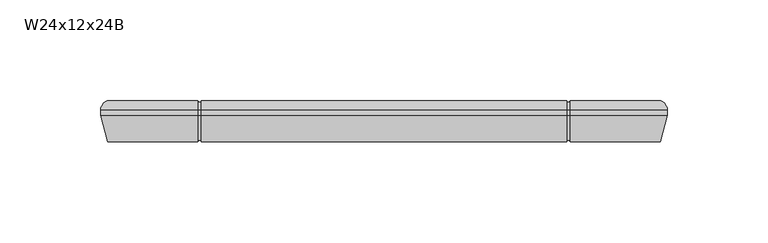
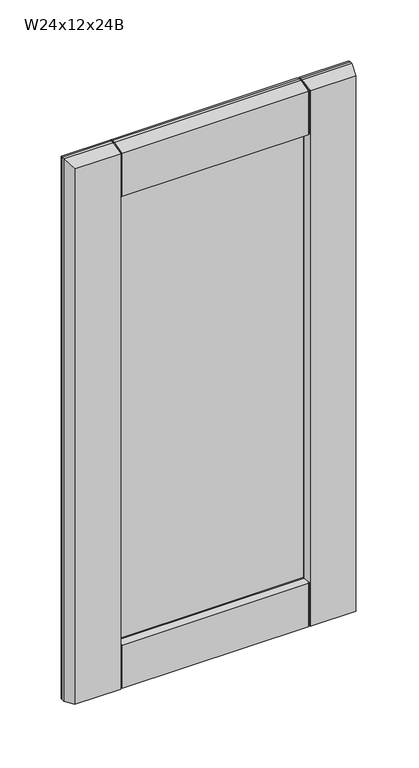
"""IFC4 building model written with IfcOpenShell, lengths in millimetres: furniture geometry, Cabinet-Wall-Merillat-Double_Door-Marlin : W24x12x24B."""

from ifc_helpers import new_model, si_unit, frame, origin, place, context, project, spatial, polyline, circle_curve, ellipse_curve, outline, extrude, source, transform, mapped, element, save
from ifc_brep_helpers import plane_surface, cylinder_surface, advanced_brep


def w24x12x24b_108fa4a6(model_context):
    return source(origin(), model_context, "Body", "SolidModel", [
        advanced_brep(
        [(541.0528392, 382.5621, 2108.2), (541.0528392, 382.5621, 1549.4), (537.9563467, 387.0325, 1552.4964925), (537.9563467, 387.0325, 2105.1035075), (541.0528392, 379.7935, 2108.2), (541.0528392, 379.7935, 1549.4), (537.5476392, 366.7125, 2104.6948), (537.5476392, 366.7125, 1552.9052), (492.8516765, 366.7125, 2059.9988372), (492.4815448, 367.50625, 2059.6287055), (490.4003857, 371.96931, 2057.5475465), (490.4003857, 371.96931, 1600.0524535), (492.4815448, 367.50625, 1597.9712945), (492.8516765, 366.7125, 1597.6011628), (491.8001552, 374.2094093, 2058.947316), (491.8001552, 374.2094093, 1598.652684), (506.1278392, 374.4595, 2073.275), (506.1278392, 374.4595, 1584.325), (506.1278392, 379.2855, 2073.275), (506.1278392, 379.2855, 1584.325), (491.8001552, 379.5355907, 2058.947316), (491.8001552, 379.5355907, 1598.652684), (490.4003857, 381.77569, 2057.5475465), (490.4003857, 381.77569, 1600.0524535), (492.4815448, 386.23875, 2059.6287055), (492.848809, 387.0263508, 2059.9959698), (492.8516765, 387.0325, 1597.6011628), (492.4815448, 386.23875, 1597.9712945), (263.1618317, 387.0325, 1552.4964925), (308.2295579, 387.0325, 1552.4964925), (308.2295579, 382.5621, 1549.4), (260.0653392, 382.5621, 1549.4), (492.848809, 382.5621, 1549.4), (492.848809, 387.0325, 1552.4964925), (491.261309, 382.5621, 1549.4), (309.8170579, 382.5621, 1549.4), (309.8170579, 387.0325, 1552.4964925), (491.261309, 387.0325, 1552.4964925), (308.2295579, 379.7935, 1549.4), (260.0653392, 379.7935, 1549.4), (492.848809, 379.7935, 1549.4), (491.261309, 379.7935, 1549.4), (309.8170579, 379.7935, 1549.4), (308.2295579, 366.7125, 1552.9052), (263.5705392, 366.7125, 1552.9052), (491.261309, 366.7125, 1552.9052), (309.8170579, 366.7125, 1552.9052), (492.848809, 366.7125, 1552.9052), (310.7177927, 371.96931, 1600.0524535), (308.6366337, 367.50625, 1597.9712945), (309.8170579, 367.50625, 1597.9712945), (309.8170579, 366.7125, 1597.6011628), (491.261309, 366.7125, 1597.6011628), (491.261309, 367.50625, 1597.9712945), (309.3180233, 374.2094093, 1598.652684), (294.9903392, 374.4595, 1584.325), (294.9903392, 379.2855, 1584.325), (309.3180233, 379.5355907, 1598.652684), (310.7177927, 381.77569, 1600.0524535), (491.261309, 386.23875, 1597.9712945), (491.261309, 387.0325, 1597.6011628), (309.8170579, 387.0325, 1597.6011628), (309.8170579, 386.23875, 1597.9712945), (308.6366337, 386.23875, 1597.9712945), (260.0653392, 382.5621, 2108.2), (263.1618317, 387.0325, 2105.1035075), (260.0653392, 379.7935, 2108.2), (263.5705392, 366.7125, 2104.6948), (308.266502, 366.7125, 1597.6011628), (310.7177927, 371.96931, 2057.5475465), (308.6366337, 367.50625, 2059.6287055), (308.266502, 366.7125, 2059.9988372), (309.3180233, 374.2094093, 2058.947316), (294.9903392, 374.4595, 2073.275), (294.9903392, 379.2855, 2073.275), (309.3180233, 379.5355907, 2058.947316), (310.7177927, 381.77569, 2057.5475465), (308.266502, 387.0325, 1597.6011628), (308.266502, 387.0325, 2059.9988372), (308.6366337, 386.23875, 2059.6287055), (492.848809, 387.0325, 2105.1035075), (492.848809, 382.5621, 2108.2), (308.2295579, 382.5621, 2108.2), (308.2295579, 387.0325, 2105.1035075), (309.8170579, 382.5621, 2108.2), (491.261309, 382.5621, 2108.2), (491.261309, 387.0325, 2105.1035075), (309.8170579, 387.0325, 2105.1035075), (492.848809, 379.7935, 2108.2), (308.2295579, 379.7935, 2108.2), (309.8170579, 379.7935, 2108.2), (491.261309, 379.7935, 2108.2), (492.848809, 366.7125, 2104.6948), (308.2295579, 366.7125, 2104.6948), (309.8170579, 366.7125, 2104.6948), (491.261309, 366.7125, 2104.6948), (309.8170579, 366.7125, 2059.9988372), (491.261309, 366.7125, 2059.9988372), (491.261309, 367.50625, 2059.6287055), (309.8170579, 367.50625, 2059.6287055), (309.8170579, 386.23875, 2059.6287055), (309.8170579, 387.0325, 2059.9988372), (491.261309, 387.0325, 2059.9988372), (491.261309, 386.23875, 2059.6287055), (309.8170579, 386.23875, 2104.9526052), (309.8170579, 382.5621, 2107.40625), (309.8170579, 379.8980037, 2107.40625), (309.8170579, 367.50625, 2104.0857412), (308.2295579, 367.50625, 2059.6287055), (308.2295579, 367.50625, 2104.0857412), (308.2295579, 379.8980037, 2107.40625), (308.2295579, 382.5621, 2107.40625), (308.2295579, 386.23875, 2104.9526052), (308.2295579, 386.23875, 2059.6287055), (492.848809, 386.23875, 2059.6287055), (492.848809, 386.23875, 2104.9526052), (492.848809, 382.5621, 2107.40625), (492.848809, 379.8980037, 2107.40625), (492.848809, 367.50625, 2104.0857412), (492.848809, 367.50625, 2059.6287055), (491.261309, 367.50625, 2104.0857412), (491.261309, 379.8980037, 2107.40625), (491.261309, 382.5621, 2107.40625), (491.261309, 386.23875, 2104.9526052), (492.848809, 367.50625, 1597.9712945), (492.848809, 367.50625, 1553.5142588), (492.848809, 379.8980037, 1550.19375), (492.848809, 382.5621, 1550.19375), (492.848809, 386.23875, 1552.6473948), (492.848809, 386.23875, 1597.9712945), (491.261309, 386.23875, 1552.6473948), (491.261309, 382.5621, 1550.19375), (491.261309, 379.8980037, 1550.19375), (491.261309, 367.50625, 1553.5142588), (309.8170579, 367.50625, 1553.5142588), (309.8170579, 379.8980037, 1550.19375), (309.8170579, 382.5621, 1550.19375), (309.8170579, 386.23875, 1552.6473948), (308.2295579, 386.23875, 1597.9712945), (308.2295579, 386.23875, 1552.6473948), (308.2295579, 382.5621, 1550.19375), (308.2295579, 379.8980037, 1550.19375), (308.2295579, 367.50625, 1553.5142588), (308.2295579, 367.50625, 1597.9712945)],
        [
            (0, 1),
            (1, 2, ellipse_curve(frame((536.2776392, 382.5621, 1554.1752), z_axis=(0.7071067811865475, 0.0, 0.7071067811865475), x_axis=(-0.7071067811865474, 0.0, 0.7071067811865476)), 6.7531526, 4.7752)),
            (2, 3),
            (3, 0, ellipse_curve(frame((536.2776392, 382.5621, 2103.4248), z_axis=(0.7071067811865475, 0.0, -0.7071067811865475), x_axis=(0.7071067811865474, 0.0, 0.7071067811865476)), 6.7531526, 4.7752)),
            (0, 4),
            (4, 5),
            (5, 1),
            (4, 6),
            (6, 7),
            (7, 5),
            (8, 9),
            (9, 10),
            (10, 11),
            (11, 12),
            (12, 13),
            (13, 8),
            (10, 14, ellipse_curve(frame((491.8276392, 372.6348492, 2058.9748), z_axis=(0.7071067811865475, 0.0, -0.7071067811865475), x_axis=(0.7071067811865474, 0.0, 0.7071067811865476)), 2.2271035, 1.5748)),
            (14, 15),
            (15, 11, ellipse_curve(frame((491.8276392, 372.6348492, 1598.6252), z_axis=(0.7071067811865475, 0.0, 0.7071067811865475), x_axis=(-0.7071067811865474, 0.0, 0.7071067811865476)), 2.2271035, 1.5748)),
            (14, 16),
            (16, 17),
            (17, 15),
            (16, 18),
            (18, 19),
            (19, 17),
            (18, 20),
            (20, 21),
            (21, 19),
            (20, 22, ellipse_curve(frame((491.8276392, 381.1101508, 2058.9748), z_axis=(0.7071067811865475, 0.0, -0.7071067811865475), x_axis=(0.7071067811865474, 0.0, 0.7071067811865476)), 2.2271035, 1.5748)),
            (22, 23),
            (23, 21, ellipse_curve(frame((491.8276392, 381.1101508, 1598.6252), z_axis=(0.7071067811865475, 0.0, 0.7071067811865475), x_axis=(-0.7071067811865474, 0.0, 0.7071067811865476)), 2.2271035, 1.5748)),
            (22, 24),
            (24, 25),
            (25, 26),
            (26, 27),
            (27, 23),
            (28, 29),
            (29, 30, circle_curve(frame((308.2295579, 382.5621, 1554.1752), z_axis=(-1.0, 0.0, 0.0), x_axis=(0.0, -1.0, 0.0)), 4.7752)),
            (30, 31),
            (31, 28, ellipse_curve(frame((264.8405392, 382.5621, 1554.1752), z_axis=(0.7071067811865475, 0.0, -0.7071067811865475), x_axis=(0.7071067811865476, 0.0, 0.7071067811865474)), 6.7531526, 4.7752)),
            (1, 32),
            (32, 33, circle_curve(frame((492.848809, 382.5621, 1554.1752), z_axis=(1.0, 0.0, 0.0), x_axis=(0.0, -1.0, 0.0)), 4.7752)),
            (33, 2),
            (34, 35),
            (35, 36, circle_curve(frame((309.8170579, 382.5621, 1554.1752), z_axis=(1.0, 0.0, 0.0), x_axis=(0.0, -1.0, 0.0)), 4.7752)),
            (36, 37),
            (37, 34, circle_curve(frame((491.261309, 382.5621, 1554.1752), z_axis=(-1.0, 0.0, 0.0), x_axis=(0.0, -1.0, 0.0)), 4.7752)),
            (30, 38),
            (38, 39),
            (39, 31),
            (5, 40),
            (40, 32),
            (41, 42),
            (42, 35),
            (34, 41),
            (38, 43),
            (43, 44),
            (44, 39),
            (45, 46),
            (46, 42),
            (41, 45),
            (7, 47),
            (47, 40),
            (48, 49),
            (49, 50),
            (50, 51),
            (51, 52),
            (52, 53),
            (53, 12),
            (11, 48),
            (15, 54),
            (54, 48, ellipse_curve(frame((309.2905392, 372.6348492, 1598.6252), z_axis=(0.7071067811865475, 0.0, -0.7071067811865475), x_axis=(0.7071067811865476, 0.0, 0.7071067811865474)), 2.2271035, 1.5748)),
            (17, 55),
            (55, 54),
            (19, 56),
            (56, 55),
            (21, 57),
            (57, 56),
            (23, 58),
            (58, 57, ellipse_curve(frame((309.2905392, 381.1101508, 1598.6252), z_axis=(0.7071067811865475, 0.0, -0.7071067811865475), x_axis=(0.7071067811865476, 0.0, 0.7071067811865474)), 2.2271035, 1.5748)),
            (27, 59),
            (59, 60),
            (60, 61),
            (61, 62),
            (62, 63),
            (63, 58),
            (31, 64),
            (64, 65, ellipse_curve(frame((264.8405392, 382.5621, 2103.4248), z_axis=(-0.7071067811865475, 0.0, -0.7071067811865475), x_axis=(0.7071067811865474, 0.0, -0.7071067811865476)), 6.7531526, 4.7752)),
            (65, 28),
            (39, 66),
            (66, 64),
            (44, 67),
            (67, 66),
            (68, 49),
            (48, 69),
            (69, 70),
            (70, 71),
            (71, 68),
            (54, 72),
            (72, 69, ellipse_curve(frame((309.2905392, 372.6348492, 2058.9748), z_axis=(-0.7071067811865475, 0.0, -0.7071067811865475), x_axis=(0.7071067811865474, 0.0, -0.7071067811865476)), 2.2271035, 1.5748)),
            (55, 73),
            (73, 72),
            (56, 74),
            (74, 73),
            (57, 75),
            (75, 74),
            (58, 76),
            (76, 75, ellipse_curve(frame((309.2905392, 381.1101508, 2058.9748), z_axis=(-0.7071067811865475, 0.0, -0.7071067811865475), x_axis=(0.7071067811865474, 0.0, -0.7071067811865476)), 2.2271035, 1.5748)),
            (63, 77),
            (77, 78),
            (78, 79),
            (79, 76),
            (3, 80),
            (80, 81, circle_curve(frame((492.848809, 382.5621, 2103.4248), z_axis=(1.0, 0.0, 0.0), x_axis=(0.0, -1.0, 0.0)), 4.7752)),
            (81, 0),
            (64, 82),
            (82, 83, circle_curve(frame((308.2295579, 382.5621, 2103.4248), z_axis=(-1.0, 0.0, 0.0), x_axis=(0.0, -1.0, 0.0)), 4.7752)),
            (83, 65),
            (84, 85),
            (85, 86, circle_curve(frame((491.261309, 382.5621, 2103.4248), z_axis=(-1.0, 0.0, 0.0), x_axis=(0.0, -1.0, 0.0)), 4.7752)),
            (86, 87),
            (87, 84, circle_curve(frame((309.8170579, 382.5621, 2103.4248), z_axis=(1.0, 0.0, 0.0), x_axis=(0.0, -1.0, 0.0)), 4.7752)),
            (81, 88),
            (88, 4),
            (66, 89),
            (89, 82),
            (90, 91),
            (91, 85),
            (84, 90),
            (88, 92),
            (92, 6),
            (67, 93),
            (93, 89),
            (94, 95),
            (95, 91),
            (90, 94),
            (51, 46),
            (45, 52),
            (43, 68),
            (71, 93),
            (92, 8),
            (13, 47),
            (96, 97),
            (97, 95),
            (94, 96),
            (9, 98),
            (98, 97),
            (96, 99),
            (99, 70),
            (69, 10),
            (72, 14),
            (73, 16),
            (74, 18),
            (75, 20),
            (76, 22),
            (79, 100),
            (100, 101),
            (101, 102),
            (102, 103),
            (103, 24),
            (33, 26),
            (25, 80),
            (36, 61),
            (60, 37),
            (83, 78),
            (77, 29),
            (86, 102),
            (101, 87),
            (100, 104),
            (104, 105, circle_curve(frame((309.8170579, 382.5621, 2103.4248), z_axis=(1.0, 0.0, 0.0), x_axis=(0.0, 0.0, 1.0)), 3.98145)),
            (105, 106),
            (106, 107),
            (107, 99),
            (71, 108),
            (108, 109),
            (109, 110),
            (110, 111),
            (111, 112, circle_curve(frame((308.2295579, 382.5621, 2103.4248), z_axis=(-1.0, 0.0, 0.0), x_axis=(0.0, 0.0, 1.0)), 3.98145)),
            (112, 113),
            (113, 78),
            (113, 79),
            (112, 104),
            (111, 105),
            (110, 106),
            (109, 107),
            (108, 70),
            (25, 114),
            (114, 115),
            (115, 116, circle_curve(frame((492.848809, 382.5621, 2103.4248), z_axis=(1.0, 0.0, 0.0), x_axis=(0.0, 0.0, 1.0)), 3.98145)),
            (116, 117),
            (117, 118),
            (118, 119),
            (119, 8),
            (98, 120),
            (120, 121),
            (121, 122),
            (122, 123, circle_curve(frame((491.261309, 382.5621, 2103.4248), z_axis=(-1.0, 0.0, 0.0), x_axis=(0.0, 0.0, 1.0)), 3.98145)),
            (123, 103),
            (24, 114),
            (123, 115),
            (122, 116),
            (121, 117),
            (120, 118),
            (9, 119),
            (13, 124),
            (124, 125),
            (125, 126),
            (126, 127),
            (127, 128, circle_curve(frame((492.848809, 382.5621, 1554.1752), z_axis=(1.0, 0.0, 0.0), x_axis=(0.0, 0.0, 1.0)), 3.98145)),
            (128, 129),
            (129, 26),
            (59, 130),
            (130, 131, circle_curve(frame((491.261309, 382.5621, 1554.1752), z_axis=(-1.0, 0.0, 0.0), x_axis=(0.0, 0.0, 1.0)), 3.98145)),
            (131, 132),
            (132, 133),
            (133, 53),
            (12, 124),
            (133, 125),
            (132, 126),
            (131, 127),
            (130, 128),
            (27, 129),
            (50, 134),
            (134, 135),
            (135, 136),
            (136, 137, circle_curve(frame((309.8170579, 382.5621, 1554.1752), z_axis=(1.0, 0.0, 0.0), x_axis=(0.0, 0.0, 1.0)), 3.98145)),
            (137, 62),
            (138, 139),
            (139, 140, circle_curve(frame((308.2295579, 382.5621, 1554.1752), z_axis=(-1.0, 0.0, 0.0), x_axis=(0.0, 0.0, 1.0)), 3.98145)),
            (140, 141),
            (141, 142),
            (142, 143),
            (143, 68),
            (77, 138),
            (63, 138),
            (143, 49),
            (142, 134),
            (141, 135),
            (140, 136),
            (139, 137),
        ],
        [
            cylinder_surface(frame((536.2776392, 382.5621, 2108.2), z_axis=(0.0, 0.0, 1.0), x_axis=(0.0, -1.0, 0.0)), 4.7752),
            plane_surface(frame((541.0528392, 382.5621, 2108.2), z_axis=(1.0, 0.0, 0.0), x_axis=(0.0, 0.0, -1.0))),
            plane_surface(frame((541.0528392, 379.7935, 2108.2), z_axis=(0.9659229350723619, -0.25882983502910506, 0.0), x_axis=(0.0, 0.0, -1.0))),
            plane_surface(frame((492.8516765, 366.7125, 2059.9988372), z_axis=(-0.9063077870366099, -0.4226182617407856, 0.0), x_axis=(0.0, 0.0, -1.0))),
            cylinder_surface(frame((491.8276392, 372.6348492, 2108.2), z_axis=(0.0, 0.0, 1.0000000000000002), x_axis=(-0.01745240643729364, 0.9998476951563912, 0.0)), 1.5748),
            plane_surface(frame((491.8001552, 374.2094093, 2058.947316), z_axis=(-0.017452406437322144, 0.9998476951563906, 0.0), x_axis=(0.0, 0.0, -1.0))),
            plane_surface(frame((506.1278392, 374.4595, 2073.275), z_axis=(-1.0, 0.0, 0.0), x_axis=(0.0, 0.0, -1.0))),
            plane_surface(frame((506.1278392, 379.2855, 2073.275), z_axis=(-0.01745240643727848, -0.9998476951563914, 0.0), x_axis=(0.0, 0.0, -1.0))),
            cylinder_surface(frame((491.8276392, 381.1101508, 2108.2), z_axis=(0.0, 0.0, 1.0000000000000002), x_axis=(-0.9063077870367326, 0.42261826174052236, 0.0)), 1.5748),
            plane_surface(frame((490.4003857, 381.77569, 2057.5475465), z_axis=(-0.9063077870366333, 0.4226182617407352, 0.0), x_axis=(0.0, 0.0, -1.0))),
            cylinder_surface(frame((541.0528392, 382.5621, 1554.1752), z_axis=(1.0, 0.0, 0.0), x_axis=(0.0, -1.0, 0.0)), 4.7752),
            plane_surface(frame((541.0528392, 382.5621, 1549.4), z_axis=(0.0, 0.0, -1.0), x_axis=(-1.0, 0.0, 0.0))),
            plane_surface(frame((541.0528392, 379.7935, 1549.4), z_axis=(0.0, -0.2588298350291095, -0.9659229350723607), x_axis=(-1.0, 0.0, 0.0))),
            plane_surface(frame((492.8516765, 366.7125, 1597.6011628), z_axis=(0.0, -0.42261826174078143, 0.9063077870366119), x_axis=(-1.0, 0.0, 0.0))),
            cylinder_surface(frame((541.0528392, 372.6348492, 1598.6252), z_axis=(1.0000000000000002, 0.0, 0.0), x_axis=(0.0, 0.9998476951563913, 0.017452406437289025)), 1.5748),
            plane_surface(frame((491.8001552, 374.2094093, 1598.652684), z_axis=(0.0, 0.9998476951563907, 0.01745240643731753), x_axis=(-1.0, 0.0, 0.0))),
            plane_surface(frame((506.1278392, 374.4595, 1584.325), z_axis=(0.0, 0.0, 1.0), x_axis=(-1.0, 0.0, 0.0))),
            plane_surface(frame((506.1278392, 379.2855, 1584.325), z_axis=(0.0, -0.9998476951563913, 0.017452406437283095), x_axis=(-1.0, 0.0, 0.0))),
            cylinder_surface(frame((541.0528392, 381.1101508, 1598.6252), z_axis=(1.0000000000000002, 0.0, 0.0), x_axis=(0.0, 0.4226182617405265, 0.9063077870367306)), 1.5748),
            plane_surface(frame((490.4003857, 381.77569, 1600.0524535), z_axis=(0.0, 0.4226182617407394, 0.9063077870366314), x_axis=(-1.0, 0.0, 0.0))),
            cylinder_surface(frame((264.8405392, 382.5621, 1549.4), z_axis=(0.0, 0.0, -1.0), x_axis=(0.0, -1.0, 0.0)), 4.7752),
            plane_surface(frame((260.0653392, 382.5621, 1549.4), z_axis=(-1.0, 0.0, 0.0), x_axis=(0.0, 0.0, 1.0))),
            plane_surface(frame((260.0653392, 379.7935, 1549.4), z_axis=(-0.9659229350723619, -0.25882983502910506, 0.0), x_axis=(0.0, 0.0, 1.0))),
            plane_surface(frame((308.266502, 366.7125, 1597.6011628), z_axis=(0.9063077870366099, -0.4226182617407856, 0.0), x_axis=(0.0, 0.0, 1.0))),
            cylinder_surface(frame((309.2905392, 372.6348492, 1549.4), z_axis=(0.0, 0.0, -1.0000000000000002), x_axis=(0.01745240643729364, 0.9998476951563912, 0.0)), 1.5748),
            plane_surface(frame((309.3180233, 374.2094093, 1598.652684), z_axis=(0.017452406437322144, 0.9998476951563906, 0.0), x_axis=(0.0, 0.0, 1.0))),
            plane_surface(frame((294.9903392, 374.4595, 1584.325), z_axis=(1.0, 0.0, 0.0), x_axis=(0.0, 0.0, 1.0))),
            plane_surface(frame((294.9903392, 379.2855, 1584.325), z_axis=(0.01745240643727848, -0.9998476951563914, 0.0), x_axis=(0.0, 0.0, 1.0))),
            cylinder_surface(frame((309.2905392, 381.1101508, 1549.4), z_axis=(0.0, 0.0, -1.0000000000000002), x_axis=(0.9063077870367326, 0.42261826174052236, 0.0)), 1.5748),
            plane_surface(frame((310.7177927, 381.77569, 1600.0524535), z_axis=(0.9063077870366333, 0.4226182617407352, 0.0), x_axis=(0.0, 0.0, 1.0))),
            cylinder_surface(frame((260.0653392, 382.5621, 2103.4248), z_axis=(-1.0, 0.0, 0.0), x_axis=(0.0, -1.0, 0.0)), 4.7752),
            plane_surface(frame((260.0653392, 382.5621, 2108.2), z_axis=(0.0, 0.0, 1.0), x_axis=(1.0, 0.0, 0.0))),
            plane_surface(frame((260.0653392, 379.7935, 2108.2), z_axis=(0.0, -0.2588298350291006, 0.9659229350723632), x_axis=(1.0, 0.0, 0.0))),
            plane_surface(frame((263.5705392, 366.7125, 2104.6948), z_axis=(0.0, -1.0, 0.0), x_axis=(1.0, 0.0, 0.0))),
            plane_surface(frame((308.266502, 366.7125, 2059.9988372), z_axis=(0.0, -0.42261826174078976, -0.9063077870366079), x_axis=(1.0, 0.0, 0.0))),
            cylinder_surface(frame((260.0653392, 372.6348492, 2058.9748), z_axis=(-1.0000000000000002, 0.0, 0.0), x_axis=(0.0, 0.999847695156391, -0.017452406437298253)), 1.5748),
            plane_surface(frame((309.3180233, 374.2094093, 2058.947316), z_axis=(0.0, 0.9998476951563905, -0.01745240643732676), x_axis=(1.0, 0.0, 0.0))),
            plane_surface(frame((294.9903392, 374.4595, 2073.275), z_axis=(0.0, 0.0, -1.0), x_axis=(1.0, 0.0, 0.0))),
            plane_surface(frame((294.9903392, 379.2855, 2073.275), z_axis=(0.0, -0.9998476951563915, -0.017452406437273867), x_axis=(1.0, 0.0, 0.0))),
            cylinder_surface(frame((260.0653392, 381.1101508, 2058.9748), z_axis=(-1.0000000000000002, 0.0, 0.0), x_axis=(0.0, 0.4226182617405182, -0.9063077870367346)), 1.5748),
            plane_surface(frame((310.7177927, 381.77569, 2057.5475465), z_axis=(0.0, 0.422618261740731, -0.9063077870366353), x_axis=(1.0, 0.0, 0.0))),
            plane_surface(frame((308.266502, 387.0325, 2059.9988372), z_axis=(0.0, 1.0, 0.0), x_axis=(1.0, 0.0, 0.0))),
            plane_surface(frame((309.8170579, 387.0325, 2059.9988372), z_axis=(-1.0000000000000002, 0.0, 0.0), x_axis=(0.0, -0.9063077870366395, -0.42261826174072203))),
            plane_surface(frame((308.2295579, 387.0325, 2059.9988372), z_axis=(1.0000000000000002, 0.0, 0.0), x_axis=(0.0, 0.9063077870366395, 0.42261826174072203))),
            plane_surface(frame((309.8170579, 387.0325, 2059.9988372), z_axis=(0.0, -0.42261826174072203, 0.9063077870366395), x_axis=(-1.0, 0.0, 0.0))),
            plane_surface(frame((309.8170579, 386.23875, 2059.6287055), z_axis=(0.0, 1.0, 0.0), x_axis=(-1.0, 0.0, 0.0))),
            cylinder_surface(frame((308.2295579, 382.5621, 2103.4248), z_axis=(-1.0, 0.0, 0.0), x_axis=(0.0, 0.0, 1.0)), 3.98145),
            plane_surface(frame((309.8170579, 382.5621, 2107.40625), z_axis=(0.0, 0.0, 1.0), x_axis=(-1.0, 0.0, 0.0))),
            plane_surface(frame((309.8170579, 379.8980037, 2107.40625), z_axis=(0.0, -0.25882983502916385, 0.9659229350723462), x_axis=(-1.0, 0.0, 0.0))),
            plane_surface(frame((309.8170579, 367.50625, 2104.0857412), z_axis=(0.0, -1.0, 0.0), x_axis=(-1.0, 0.0, 0.0))),
            plane_surface(frame((309.8170579, 367.50625, 2059.6287055), z_axis=(0.0, 0.4226182617407834, 0.9063077870366109), x_axis=(-1.0, 0.0, 0.0))),
            plane_surface(frame((492.848809, 387.0325, 2059.9988372), z_axis=(-1.0, 0.0, 0.0), x_axis=(0.0, -0.9063077870366473, -0.4226182617407054))),
            plane_surface(frame((491.261309, 387.0325, 2059.9988372), z_axis=(1.0, 0.0, 0.0), x_axis=(0.0, 0.9063077870366473, 0.4226182617407054))),
            plane_surface(frame((492.848809, 387.0325, 2059.9988372), z_axis=(0.0, -0.4226182617407054, 0.9063077870366473), x_axis=(-1.0, 0.0, 0.0))),
            plane_surface(frame((492.848809, 386.23875, 2059.6287055), z_axis=(0.0, 1.0, 0.0), x_axis=(-1.0, 0.0, 0.0))),
            cylinder_surface(frame((491.261309, 382.5621, 2103.4248), z_axis=(-1.0, 0.0, 0.0), x_axis=(0.0, 0.0, 1.0)), 3.98145),
            plane_surface(frame((492.848809, 382.5621, 2107.40625), z_axis=(0.0, 0.0, 1.0), x_axis=(-1.0, 0.0, 0.0))),
            plane_surface(frame((492.848809, 379.8980037, 2107.40625), z_axis=(0.0, -0.2588298350291636, 0.9659229350723463), x_axis=(-1.0, 0.0, 0.0))),
            plane_surface(frame((492.848809, 367.50625, 2104.0857412), z_axis=(0.0, -1.0, 0.0), x_axis=(-1.0, 0.0, 0.0))),
            plane_surface(frame((492.848809, 367.50625, 2059.6287055), z_axis=(0.0, 0.4226182617407987, 0.9063077870366038), x_axis=(-1.0, 0.0, 0.0))),
            plane_surface(frame((492.848809, 382.5621, 1558.9504), z_axis=(-1.0, 0.0, 0.0), x_axis=(0.0, 1.0, 0.0))),
            plane_surface(frame((491.261309, 382.5621, 1558.9504), z_axis=(1.0, 0.0, 0.0), x_axis=(0.0, -1.0, 0.0))),
            plane_surface(frame((492.848809, 366.7125, 1597.6011628), z_axis=(0.0, 0.42261826174078765, -0.906307787036609), x_axis=(-1.0, 0.0, 0.0))),
            plane_surface(frame((492.848809, 367.50625, 1597.9712945), z_axis=(0.0, -1.0, 0.0), x_axis=(-1.0, 0.0, 0.0))),
            plane_surface(frame((492.848809, 367.50625, 1553.5142588), z_axis=(0.0, -0.25882983502943846, -0.9659229350722726), x_axis=(-1.0, 0.0, 0.0))),
            plane_surface(frame((492.848809, 379.8980037, 1550.19375), z_axis=(0.0, 0.0, -1.0), x_axis=(-1.0, 0.0, 0.0))),
            cylinder_surface(frame((491.261309, 382.5621, 1554.1752), z_axis=(-1.0, 0.0, 0.0), x_axis=(0.0, 0.0, 1.0)), 3.98145),
            plane_surface(frame((492.848809, 386.23875, 1552.6473948), z_axis=(0.0, 1.0, 0.0), x_axis=(-1.0, 0.0, 0.0))),
            plane_surface(frame((492.848809, 386.23875, 1597.9712945), z_axis=(0.0, -0.42261826174073697, -0.9063077870366324), x_axis=(-1.0, 0.0, 0.0))),
            plane_surface(frame((309.8170579, 386.23875, 1597.9712945), z_axis=(-1.0, 0.0, 0.0), x_axis=(0.0, 0.9063077870366392, -0.4226182617407227))),
            plane_surface(frame((308.2295579, 386.23875, 1597.9712945), z_axis=(1.0, 0.0, 0.0), x_axis=(0.0, -0.9063077870366392, 0.4226182617407227))),
            plane_surface(frame((309.8170579, 386.23875, 1597.9712945), z_axis=(0.0, -0.4226182617407227, -0.9063077870366392), x_axis=(-1.0, 0.0, 0.0))),
            plane_surface(frame((309.8170579, 366.7125, 1597.6011628), z_axis=(0.0, 0.42261826174079387, -0.9063077870366061), x_axis=(-1.0, 0.0, 0.0))),
            plane_surface(frame((309.8170579, 367.50625, 1597.9712945), z_axis=(0.0, -1.0, 0.0), x_axis=(-1.0, 0.0, 0.0))),
            plane_surface(frame((309.8170579, 367.50625, 1553.5142588), z_axis=(0.0, -0.2588298350294392, -0.9659229350722724), x_axis=(-1.0, 0.0, 0.0))),
            plane_surface(frame((309.8170579, 379.8980037, 1550.19375), z_axis=(0.0, 0.0, -1.0), x_axis=(-1.0, 0.0, 0.0))),
            cylinder_surface(frame((308.2295579, 382.5621, 1554.1752), z_axis=(-1.0, 0.0, 0.0), x_axis=(0.0, 0.0, 1.0)), 3.98145),
            plane_surface(frame((309.8170579, 386.23875, 1552.6473948), z_axis=(0.0, 1.0, 0.0), x_axis=(-1.0, 0.0, 0.0))),
        ],
        [
            (0, [[1, 2, 3, 4]]),
            (1, [[5, 6, 7, -1]]),
            (2, [[8, 9, 10, -6]]),
            (3, [[11, 12, 13, 14, 15, 16]]),
            (4, [[17, 18, 19, -13]]),
            (5, [[20, 21, 22, -18]]),
            (6, [[23, 24, 25, -21]]),
            (7, [[26, 27, 28, -24]]),
            (8, [[29, 30, 31, -27]]),
            (9, [[32, 33, 34, 35, 36, -30]]),
            (10, [[37, 38, 39, 40]]),
            (10, [[41, 42, 43, -2]]),
            (10, [[44, 45, 46, 47]]),
            (11, [[-39, 48, 49, 50]]),
            (11, [[51, 52, -41, -7]]),
            (11, [[53, 54, -44, 55]]),
            (12, [[-49, 56, 57, 58]]),
            (12, [[59, 60, -53, 61]]),
            (12, [[62, 63, -51, -10]]),
            (13, [[64, 65, 66, 67, 68, 69, -14, 70]]),
            (14, [[71, 72, -70, -19]]),
            (15, [[73, 74, -71, -22]]),
            (16, [[75, 76, -73, -25]]),
            (17, [[77, 78, -75, -28]]),
            (18, [[79, 80, -77, -31]]),
            (19, [[-36, 81, 82, 83, 84, 85, 86, -79]]),
            (20, [[87, 88, 89, -40]]),
            (21, [[90, 91, -87, -50]]),
            (22, [[92, 93, -90, -58]]),
            (23, [[94, -64, 95, 96, 97, 98]]),
            (24, [[99, 100, -95, -72]]),
            (25, [[101, 102, -99, -74]]),
            (26, [[103, 104, -101, -76]]),
            (27, [[105, 106, -103, -78]]),
            (28, [[107, 108, -105, -80]]),
            (29, [[-86, 109, 110, 111, 112, -107]]),
            (30, [[113, 114, 115, -4]]),
            (30, [[116, 117, 118, -88]]),
            (30, [[119, 120, 121, 122]]),
            (31, [[-115, 123, 124, -5]]),
            (31, [[125, 126, -116, -91]]),
            (31, [[127, 128, -119, 129]]),
            (32, [[-124, 130, 131, -8]]),
            (32, [[132, 133, -125, -93]]),
            (32, [[134, 135, -127, 136]]),
            (33, [[-67, 137, -59, 138]]),
            (33, [[-57, 139, -98, 140, -132, -92]]),
            (33, [[-131, 141, -16, 142, -62, -9]]),
            (33, [[143, 144, -134, 145]]),
            (34, [[-12, 146, 147, -143, 148, 149, -96, 150]]),
            (35, [[-150, -100, 151, -17]]),
            (36, [[-151, -102, 152, -20]]),
            (37, [[-152, -104, 153, -23]]),
            (38, [[-153, -106, 154, -26]]),
            (39, [[-154, -108, 155, -29]]),
            (40, [[-112, 156, 157, 158, 159, 160, -32, -155]]),
            (41, [[-43, 161, -34, 162, -113, -3]]),
            (41, [[-46, 163, -83, 164]]),
            (41, [[-118, 165, -110, 166, -37, -89]]),
            (41, [[-121, 167, -158, 168]]),
            (42, [[-148, -145, -136, -129, -122, -168, -157, 169, 170, 171, 172, 173]]),
            (43, [[-165, -117, -126, -133, -140, 174, 175, 176, 177, 178, 179, 180]]),
            (44, [[181, -111, -180]]),
            (45, [[-156, -181, -179, 182, -169]]),
            (46, [[-182, -178, 183, -170]]),
            (47, [[-183, -177, 184, -171]]),
            (48, [[-184, -176, 185, -172]]),
            (49, [[-185, -175, 186, -149, -173]]),
            (50, [[-97, -186, -174]]),
            (51, [[-141, -130, -123, -114, -162, 187, 188, 189, 190, 191, 192, 193]]),
            (52, [[-159, -167, -120, -128, -135, -144, -147, 194, 195, 196, 197, 198]]),
            (53, [[-33, 199, -187]]),
            (54, [[-199, -160, -198, 200, -188]]),
            (55, [[-200, -197, 201, -189]]),
            (56, [[-201, -196, 202, -190]]),
            (57, [[-202, -195, 203, -191]]),
            (58, [[-203, -194, -146, 204, -192]]),
            (59, [[-204, -11, -193]]),
            (60, [[-161, -42, -52, -63, -142, 205, 206, 207, 208, 209, 210, 211]]),
            (61, [[-68, -138, -61, -55, -47, -164, -82, 212, 213, 214, 215, 216]]),
            (62, [[-15, 217, -205]]),
            (63, [[-217, -69, -216, 218, -206]]),
            (64, [[-218, -215, 219, -207]]),
            (65, [[-219, -214, 220, -208]]),
            (66, [[-220, -213, 221, -209]]),
            (67, [[-221, -212, -81, 222, -210]]),
            (68, [[-222, -35, -211]]),
            (69, [[-84, -163, -45, -54, -60, -137, -66, 223, 224, 225, 226, 227]]),
            (70, [[228, 229, 230, 231, 232, 233, -139, -56, -48, -38, -166, 234]]),
            (71, [[-109, 235, -234]]),
            (72, [[236, -94, -233]]),
            (73, [[-65, -236, -232, 237, -223]]),
            (74, [[-237, -231, 238, -224]]),
            (75, [[-238, -230, 239, -225]]),
            (76, [[-239, -229, 240, -226]]),
            (77, [[-240, -228, -235, -85, -227]]),
        ],
    ),
        extrude(outline(polyline([(294.9903392, 379.2855), (506.1278392, 379.2855), (506.1278392, 374.4595), (294.9903392, 374.4595), (294.9903392, 379.2855)])), frame((0.0, 0.0, 1584.325), z_axis=(0.0, 0.0, 1.0), x_axis=(1.0, 0.0, 0.0)), (0.0, 0.0, 1.0), 488.95),
    ])


if __name__ == "__main__":
    model = new_model("IFC4")
    model_context = context("Model", 3, world=origin())
    ifc_project = project(units=[si_unit("LENGTHUNIT", "METRE", prefix="MILLI")], contexts=[model_context])
    site = spatial("IfcSite", under=ifc_project)
    building = spatial("IfcBuilding", under=site)
    placement = place(None, origin())
    w24x12x24b_shape = w24x12x24b_108fa4a6(model_context)
    element("IfcFurniture", 1, ObjectType="Cabinet-Wall-Merillat-Double_Door-Marlin : W24x12x24B", at=placement, inside=building, context=model_context, shape_type="MappedRepresentation", body=[
        mapped(w24x12x24b_shape, transform((0.0, 0.0, 0.0), x_axis=(1.0, 0.0, 0.0), y_axis=(0.0, 1.0, 0.0), z_axis=(0.0, 0.0, 1.0))),
    ])
    save(model, "model.ifc")

# Revit data of these elements
# Type "Cabinet-Wall-Merillat-Double_Door-Marlin : W24x12x24B"
#   URL = "https://www.merillat.com/"
#   Product Page URL = "https://www.merillat.com/our-products/"
#   Product Line = "Express"
#   Product Group = "Wall Cabinet"
#   Product Documentation Link = "http://merillatbusiness.com/wp-content/uploads/2014/07/Merillat_Classic_Catalog.pdf"
#   Model = "W2442B"
#   Manufacturer = "Merillat"
#   Height Note = "Actual Height of 21 inches Cabinet is 20 1/2 inches"
#   Glass Door Note = "Glass Cabinet doors are only available in specific sizes. Please refer to the catalog for this information before requesting a glass size."
#   Finish = "Wood"
#   Description = "Wall 2442 Butt Door"
#   Construction Type = "Wall Cabinet"
#   Cabinet Construction Note = "Cabinets with B suffix have BUTT doors without a center frame stile:"
#   Assembly Code = "C1030410"
#   Spacing = 0' - 1"
#   Shelving Height = 0' - 5 1/4"
#   Door Spacing = 0' - 0 1/8"
#   Cabinet Door Width = 0' - 11 1/16"
#   Cabinet Door Height = 1' - 10"
#   Depth = 1' - 0"
#   Height = 2' - 0"
#   Top Of Cabinet = 7' - 0"
#   Width = 2' - 0"
#   COBie.Type = no
#   Top and Bottom Visibility = yes
#   Partial Overlay Butt = yes
#   Partial Overlay = no
#   Number of Shelves Greater than one = 3
#   Number of Shelves = 3
#   Middle Shelf = yes
#   Full Overlay Butt = no
#   Full Overlay = no
#   Elevation Swing Line = yes
#   Door Drawer Material = Wood - Merillat - Pecan(1)
#   Cabinet Material = Wood - Merillat - Pecan(1)
#   Cabinet Door Style = element 806847
# Element 1 (IfcFurniture, "Cabinet-Wall-Merillat-Double_Door-Marlin : W24x12x24B")
#   Materials on its faces: "Wood - Merillat - Pecan(1)"
# Materials
#   "Wood - Merillat - Pecan(1)": class "Wood", colour RGB 108 67 43, transparency 0, Cost = 0
